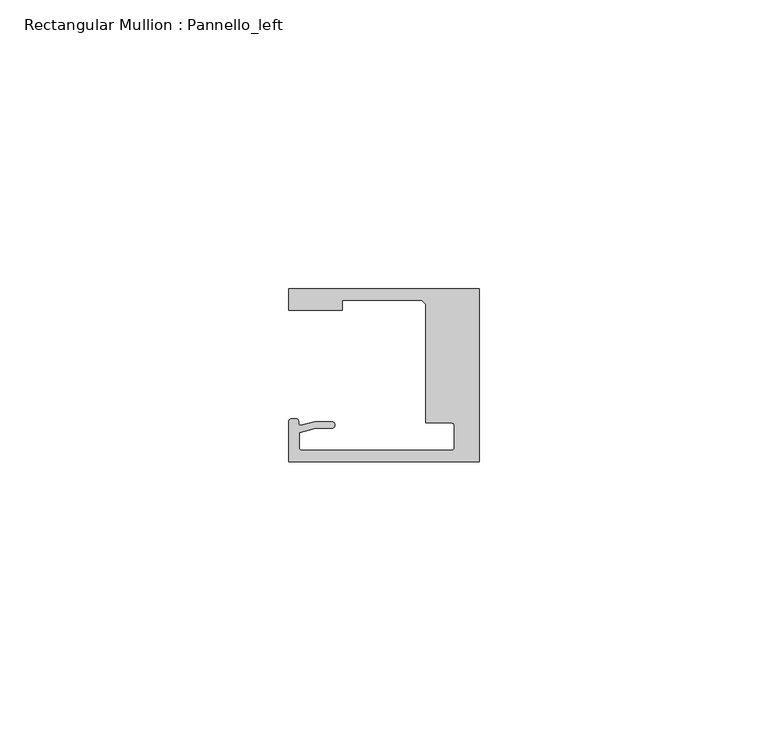
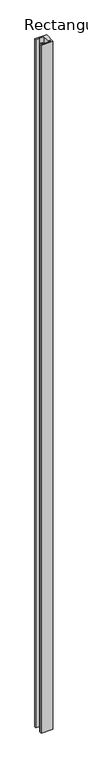
"""IFC4 building model written with IfcOpenShell, lengths in millimetres: member geometry, Rectangular Mullion : Pannello_left."""

from ifc_helpers import new_model, si_unit, frame, origin, place, context, project, spatial, polyline, circle_curve, source, transform, mapped, element, save
from ifc_brep_helpers import plane_surface, cylinder_surface, revolved_surface, extruded_surface, spline_curve, advanced_brep


def rectangular_mullion_pannello_left_b97be56f(model_context):
    return source(origin(), model_context, "Body", "AdvancedBrep", [
        advanced_brep(
        [(-33.0, 15.0, 0.0), (-33.0, 11.3000004, 0.0), (-23.700041, 11.3000004, 0.0), (-23.700041, 13.0000004, 0.0), (-10.0000103, 13.0000004, 0.0), (-9.2999726, 12.2999849, 0.0), (-9.2999726, -8.2500595, 0.0), (-4.7999726, -8.2500595, 0.0), (-4.2999726, -8.7500595, 0.0), (-4.2999726, -12.50001, 0.0), (-4.7999726, -13.00001, 0.0), (-30.69998, -13.00001, 0.0), (-31.19998, -12.50001, 0.0), (-31.19998, -9.9657591, 0.0), (-28.3419477, -9.1999523, 0.0), (-25.59998, -9.1999523, 0.0), (-25.59998, -7.9999523, 0.0), (-28.4999305, -7.9999523, 0.0), (-30.9223017, -8.6490241, 0.0), (-33.0000135, -8.0000472, 0.0), (-33.0000135, -15.0, 0.0), (0.0, -15.0, 0.0), (0.0, 15.0, 0.0), (-33.0, 15.0, -2026.9999865), (0.0, 15.0, -2026.9999865), (0.0, -15.0, -2026.9999865), (-33.0000135, -15.0, -2026.9999865), (-33.0000135, -8.0000472, -2026.9999865), (-30.9223017, -8.6490241, -2026.9999865), (-28.4999305, -7.9999523, -2026.9999865), (-25.59998, -7.9999523, -2026.9999865), (-25.59998, -9.1999523, -2026.9999865), (-28.3419477, -9.1999523, -2026.9999865), (-31.19998, -9.9657591, -2026.9999865), (-31.19998, -12.50001, -2026.9999865), (-30.69998, -13.00001, -2026.9999865), (-4.7999726, -13.00001, -2026.9999865), (-4.2999726, -12.50001, -2026.9999865), (-4.2999726, -8.7500595, -2026.9999865), (-4.7999726, -8.2500595, -2026.9999865), (-9.2999726, -8.2500595, -2026.9999865), (-9.2999726, 12.2999849, -2026.9999865), (-10.0000103, 13.0000004, -2026.9999865), (-23.700041, 13.0000004, -2026.9999865), (-23.700041, 11.3000004, -2026.9999865), (-33.0, 11.3000004, -2026.9999865)],
        [
            (0, 1),
            (1, 2),
            (2, 3),
            (3, 4),
            (4, 5),
            (5, 6),
            (6, 7),
            (7, 8, circle_curve(frame((-4.7999726, -8.7500595, 0.0), z_axis=(0.0, 0.0, -1.0), x_axis=(0.0, 1.0, 0.0)), 0.5)),
            (8, 9),
            (9, 10, circle_curve(frame((-4.7999726, -12.50001, 0.0), z_axis=(0.0, 0.0, -1.0), x_axis=(1.0, 0.0, 0.0)), 0.5)),
            (10, 11),
            (11, 12, circle_curve(frame((-30.69998, -12.50001, 0.0), z_axis=(0.0, 0.0, -1.0), x_axis=(0.0, -1.0, 0.0)), 0.5)),
            (12, 13),
            (13, 14),
            (14, 15),
            (15, 16, circle_curve(frame((-25.59998, -8.5999523, 0.0), z_axis=(0.0, 0.0, 1.0), x_axis=(0.0, -1.0, 0.0)), 0.6)),
            (16, 17),
            (17, 18),
            (18, 19, spline_curve(3, [(-30.9223017, -8.6490241, 0.0), (-31.312054066, -8.717747958, 0.0), (-31.298563602, -8.366228555, 0.0), (-31.305645054, -7.690065204, 0.0), (-31.357433266, -7.563996614, 0.0), (-32.262327879, -7.456527435, 0.0), (-33.0000135, -7.457047519, 0.0), (-33.0000135, -8.0000472, 0.0)], [4, 2, 2, 4], [0.0, 0.001840817752199412, 0.004996616814974408, 0.007702013405570312])),
            (19, 20),
            (20, 21),
            (21, 22),
            (22, 0),
            (23, 24),
            (24, 25),
            (25, 26),
            (26, 27),
            (27, 28, spline_curve(3, [(-33.0000135, -8.0000472, -2026.9999865), (-33.0000135, -7.457047519, -2026.9999865), (-32.262327879, -7.456527435, -2026.9999865), (-31.357433266, -7.563996614, -2026.9999865), (-31.305645054, -7.690065204, -2026.9999865), (-31.298563602, -8.366228555, -2026.9999865), (-31.312054066, -8.717747958, -2026.9999865), (-30.9223017, -8.6490241, -2026.9999865)], [4, 2, 2, 4], [0.0, 0.0027053965905959043, 0.0058611956533709, 0.007702013405570312])),
            (28, 29),
            (29, 30),
            (30, 31, circle_curve(frame((-25.59998, -8.5999523, -2026.9999865), z_axis=(0.0, 0.0, -1.0), x_axis=(0.0, -1.0, 0.0)), 0.6)),
            (31, 32),
            (32, 33),
            (33, 34),
            (34, 35, circle_curve(frame((-30.69998, -12.50001, -2026.9999865), z_axis=(0.0, 0.0, 1.0), x_axis=(0.0, -1.0, 0.0)), 0.5)),
            (35, 36),
            (36, 37, circle_curve(frame((-4.7999726, -12.50001, -2026.9999865), z_axis=(0.0, 0.0, 1.0), x_axis=(1.0, 0.0, 0.0)), 0.5)),
            (37, 38),
            (38, 39, circle_curve(frame((-4.7999726, -8.7500595, -2026.9999865), z_axis=(0.0, 0.0, 1.0), x_axis=(0.0, 1.0, 0.0)), 0.5)),
            (39, 40),
            (40, 41),
            (41, 42),
            (42, 43),
            (43, 44),
            (44, 45),
            (45, 23),
            (0, 23),
            (45, 1),
            (44, 2),
            (43, 3),
            (42, 4),
            (41, 5),
            (40, 6),
            (39, 7),
            (38, 8),
            (37, 9),
            (36, 10),
            (35, 11),
            (34, 12),
            (33, 13),
            (32, 14),
            (31, 15),
            (30, 16),
            (29, 17),
            (28, 18),
            (27, 19),
            (26, 20),
            (25, 21),
            (24, 22),
        ],
        [
            plane_surface(frame((0.0, -36.2491502, 0.0), z_axis=(0.0, 0.0, 1.0), x_axis=(-1.0, 0.0, 0.0))),
            plane_surface(frame((0.0, -36.2491502, -2026.9999865), z_axis=(0.0, 0.0, -1.0), x_axis=(-1.0, 0.0, 0.0))),
            plane_surface(frame((-33.0, 15.0, 0.0), z_axis=(-1.0, 0.0, 0.0), x_axis=(0.0, 0.0, -1.0))),
            plane_surface(frame((-33.0, 11.3000004, 0.0), z_axis=(0.0, -1.0, 0.0), x_axis=(0.0, 0.0, -1.0))),
            plane_surface(frame((-23.700041, 11.3000004, 0.0), z_axis=(1.0, 0.0, 0.0), x_axis=(0.0, 0.0, -1.0))),
            plane_surface(frame((-23.700041, 13.0000004, 0.0), z_axis=(0.0, -1.0, 0.0), x_axis=(0.0, 0.0, -1.0))),
            plane_surface(frame((-10.0000103, 13.0000004, 0.0), z_axis=(-0.7070955486277984, -0.7071180135668678, 0.0), x_axis=(0.0, 0.0, -1.0))),
            plane_surface(frame((-9.2999726, 12.2999849, 0.0), z_axis=(-1.0, 0.0, 0.0), x_axis=(0.0, 0.0, -1.0))),
            plane_surface(frame((-9.2999726, -8.2500595, 0.0), z_axis=(0.0, -1.0, 0.0), x_axis=(0.0, 0.0, -1.0))),
            revolved_surface(polyline([(-4.7999726, -8.2500595, -2026.9999865), (-4.7999726, -8.2500595, 0.0)]), (-4.7999726, -8.7500595, 0.0), (0.0, 0.0, -1.0)),
            plane_surface(frame((-4.2999726, -8.7500595, 0.0), z_axis=(-1.0, 0.0, 0.0), x_axis=(0.0, 0.0, -1.0))),
            revolved_surface(polyline([(-4.2999726, -12.50001, -2026.9999865), (-4.2999726, -12.50001, 0.0)]), (-4.7999726, -12.50001, 0.0), (0.0, 0.0, -1.0)),
            plane_surface(frame((-4.7999726, -13.00001, 0.0), z_axis=(0.0, 1.0, 0.0), x_axis=(0.0, 0.0, -1.0))),
            revolved_surface(polyline([(-30.69998, -13.00001, -2026.9999865), (-30.69998, -13.00001, 0.0)]), (-30.69998, -12.50001, 0.0), (0.0, 0.0, -1.0)),
            plane_surface(frame((-31.19998, -12.50001, 0.0), z_axis=(1.0, 0.0, 0.0), x_axis=(0.0, 0.0, -1.0))),
            plane_surface(frame((-31.19998, -9.9657591, 0.0), z_axis=(0.25881883204288636, -0.9659258833782002, 0.0), x_axis=(0.0, 0.0, -1.0))),
            plane_surface(frame((-28.3419477, -9.1999523, 0.0), z_axis=(0.0, -1.0, 0.0), x_axis=(0.0, 0.0, -1.0))),
            cylinder_surface(frame((-25.59998, -8.5999523, 0.0), z_axis=(0.0, 0.0, 1.0), x_axis=(0.0, -1.0, 0.0)), 0.6),
            plane_surface(frame((-25.59998, -7.9999523, 0.0), z_axis=(0.0, 1.0, 0.0), x_axis=(0.0, 0.0, -1.0))),
            plane_surface(frame((-28.4999305, -7.9999523, 0.0), z_axis=(-0.25881883200192934, 0.9659258833891746, 0.0), x_axis=(0.0, 0.0, -1.0))),
            extruded_surface(spline_curve(3, [(-30.9223017, -8.6490241, -2026.9999865), (-31.312054066, -8.717747958, -2026.9999865), (-31.298563602, -8.366228555, -2026.9999865), (-31.305645054, -7.690065204, -2026.9999865), (-31.357433266, -7.563996614, -2026.9999865), (-32.262327879, -7.456527435, -2026.9999865), (-33.0000135, -7.457047519, -2026.9999865), (-33.0000135, -8.0000472, -2026.9999865)], [4, 2, 2, 4], [0.0, 0.001840817752199412, 0.004996616814974408, 0.007702013405570312]), (0.0, 0.0, 2026.9999865), 2026.9999865),
            plane_surface(frame((-33.0000135, -8.0000472, 0.0), z_axis=(-1.0, 0.0, 0.0), x_axis=(0.0, 0.0, -1.0))),
            plane_surface(frame((-33.0000135, -15.0, 0.0), z_axis=(0.0, -1.0, 0.0), x_axis=(0.0, 0.0, -1.0))),
            plane_surface(frame((0.0, -15.0, 0.0), z_axis=(1.0, 0.0, 0.0), x_axis=(0.0, 0.0, -1.0))),
            plane_surface(frame((0.0, 15.0, 0.0), z_axis=(0.0, 1.0, 0.0), x_axis=(0.0, 0.0, -1.0))),
        ],
        [
            (0, [[1, 2, 3, 4, 5, 6, 7, 8, 9, 10, 11, 12, 13, 14, 15, 16, 17, 18, 19, 20, 21, 22, 23]]),
            (1, [[24, 25, 26, 27, 28, 29, 30, 31, 32, 33, 34, 35, 36, 37, 38, 39, 40, 41, 42, 43, 44, 45, 46]]),
            (2, [[-1, 47, -46, 48]]),
            (3, [[-2, -48, -45, 49]]),
            (4, [[-3, -49, -44, 50]]),
            (5, [[-4, -50, -43, 51]]),
            (6, [[-5, -51, -42, 52]]),
            (7, [[-6, -52, -41, 53]]),
            (8, [[-7, -53, -40, 54]]),
            (9, [[-8, -54, -39, 55]]),
            (10, [[-9, -55, -38, 56]]),
            (11, [[-10, -56, -37, 57]]),
            (12, [[-11, -57, -36, 58]]),
            (13, [[-12, -58, -35, 59]]),
            (14, [[-13, -59, -34, 60]]),
            (15, [[-14, -60, -33, 61]]),
            (16, [[-15, -61, -32, 62]]),
            (17, [[-16, -62, -31, 63]]),
            (18, [[-17, -63, -30, 64]]),
            (19, [[-18, -64, -29, 65]]),
            (20, [[-19, -65, -28, 66]]),
            (21, [[-20, -66, -27, 67]]),
            (22, [[-21, -67, -26, 68]]),
            (23, [[-22, -68, -25, 69]]),
            (24, [[-23, -69, -24, -47]]),
        ],
    ),
    ])


if __name__ == "__main__":
    model = new_model("IFC4")
    model_context = context("Model", 3, world=origin())
    ifc_project = project(units=[si_unit("LENGTHUNIT", "METRE", prefix="MILLI")], contexts=[model_context])
    site = spatial("IfcSite", under=ifc_project)
    building = spatial("IfcBuilding", under=site)
    placement = place(None, origin())
    rectangular_mullion_pannello_left_shape = rectangular_mullion_pannello_left_b97be56f(model_context)
    element("IfcMember", 1, ObjectType="Rectangular Mullion : Pannello_left", at=placement, inside=building, context=model_context, shape_type="MappedRepresentation", body=[
        mapped(rectangular_mullion_pannello_left_shape, transform((0.0, 0.0, 0.0), x_axis=(1.0, 0.0, 0.0), y_axis=(0.0, 1.0, 0.0), z_axis=(0.0, 0.0, 1.0))),
    ])
    save(model, "model.ifc")

# Revit data of these elements
# Type "Rectangular Mullion : Pannello_left"
#   built-in parameter 1007322 = 0.0984252 (stored number, unit not read)
#   built-in parameter 1007320 = 0.0305117 (stored number, unit not read)
